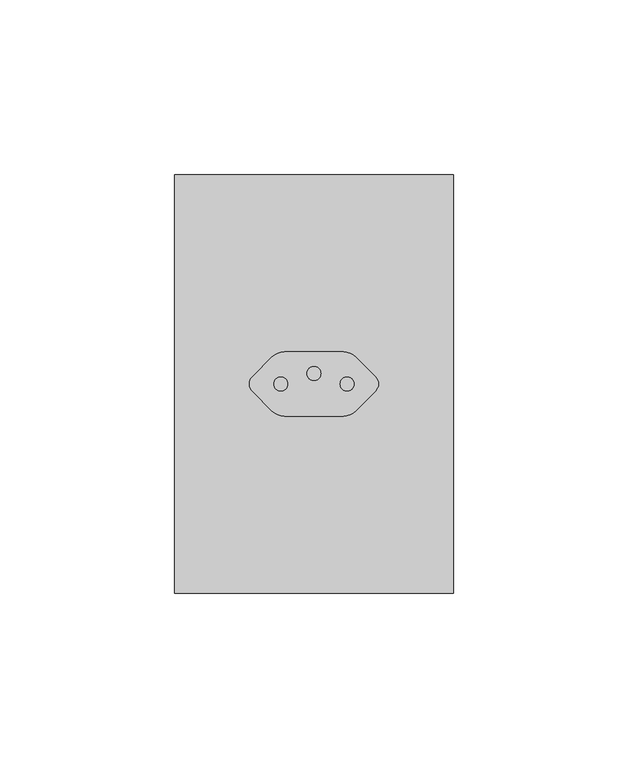
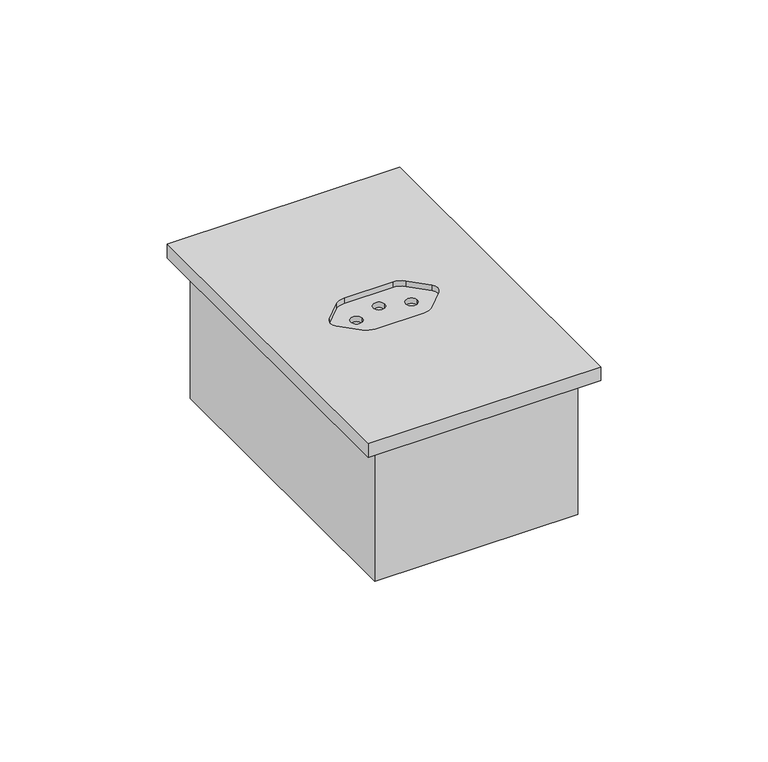
"""IFC4 building model written with IfcOpenShell, lengths in millimetres: proxy geometry, CAIXA VERTICE V7 : Tomada 10A 1s."""

from ifc_helpers import new_model, si_unit, frame, origin, place, context, project, spatial, polyline, circle_curve, faceted_brep, source, transform, mapped, element, save
from ifc_brep_helpers import plane_surface, revolved_surface, advanced_brep


def electrical_fixtures_69341c80(model_context):
    return source(origin(), model_context, "Body", "SolidModel", [
        faceted_brep([(35.0, 355.0, 0.0), (-35.0, 355.0, 0.0), (-35.0, 245.0, 0.0), (35.0, 245.0, 0.0), (33.0, 353.0, 0.0), (33.0, 247.0, 0.0), (-33.0, 247.0, 0.0), (-33.0, 353.0, 0.0), (33.0, 247.0, -48.0), (33.0, 353.0, -48.0), (-33.0, 353.0, -48.0), (-33.0, 247.0, -48.0), (35.0, 355.0, -50.0), (35.0, 245.0, -50.0), (-35.0, 245.0, -50.0), (-35.0, 355.0, -50.0)], [[[0, 1, 2, 3], [4, 5, 6, 7]], [[8, 9, 10, 11]], [[12, 13, 14, 15]], [[12, 15, 1, 0]], [[1, 15, 14, 2]], [[2, 14, 13, 3]], [[3, 13, 12, 0]], [[5, 4, 9, 8]], [[6, 5, 8, 11]], [[7, 6, 11, 10]], [[4, 7, 10, 9]]]),
        advanced_brep(
        [(40.0, 360.0, 5.0), (-40.0, 360.0, 5.0), (-40.0, 240.0, 5.0), (40.0, 240.0, 5.0), (8.4215729, 290.75, 5.0), (-8.4215729, 290.75, 5.0), (-11.9571068, 292.2144661, 5.0), (-17.6213203, 297.8786797, 5.0), (-17.6213203, 302.1213203, 5.0), (-11.9571068, 307.7855339, 5.0), (-8.4215729, 309.25, 5.0), (8.4215729, 309.25, 5.0), (11.9571068, 307.7855339, 5.0), (17.6213203, 302.1213203, 5.0), (17.6213203, 297.8786797, 5.0), (11.9571068, 292.2144661, 5.0), (-40.0, 360.0, 0.0), (40.0, 360.0, 0.0), (40.0, 240.0, 0.0), (-40.0, 240.0, 0.0), (8.4215729, 290.75, 3.0), (11.9571068, 292.2144661, 3.0), (17.6213203, 297.8786797, 3.0), (17.6213203, 302.1213203, 3.0), (11.9571068, 307.7855339, 3.0), (8.4215729, 309.25, 3.0), (-8.4215729, 309.25, 3.0), (-11.9571068, 307.7855339, 3.0), (-17.6213203, 302.1213203, 3.0), (-17.6213203, 297.8786797, 3.0), (-11.9571068, 292.2144661, 3.0), (-8.4215729, 290.75, 3.0), (-7.5, 300.0, 3.0), (-11.5, 300.0, 3.0), (11.5, 300.0, 3.0), (7.5, 300.0, 3.0), (2.0, 303.0, 3.0), (-2.0, 303.0, 3.0), (-11.5, 300.0, 1.0), (-7.5, 300.0, 1.0), (7.5, 300.0, 1.0), (11.5, 300.0, 1.0), (-2.0, 303.0, 1.0), (2.0, 303.0, 1.0)],
        [
            (0, 1),
            (1, 2),
            (2, 3),
            (3, 0),
            (4, 5),
            (5, 6, circle_curve(frame((-8.4215729, 295.75, 5.0), z_axis=(0.0, 0.0, -1.0), x_axis=(-1.0, 0.0, 0.0)), 5.0)),
            (6, 7),
            (7, 8, circle_curve(frame((-15.5, 300.0, 5.0), z_axis=(0.0, 0.0, -1.0), x_axis=(-1.0, 0.0, 0.0)), 3.0)),
            (8, 9),
            (9, 10, circle_curve(frame((-8.4215729, 304.25, 5.0), z_axis=(0.0, 0.0, -1.0), x_axis=(-1.0, 0.0, 0.0)), 5.0)),
            (10, 11),
            (11, 12, circle_curve(frame((8.4215729, 304.25, 5.0), z_axis=(0.0, 0.0, -1.0), x_axis=(-1.0, 0.0, 0.0)), 5.0)),
            (12, 13),
            (13, 14, circle_curve(frame((15.5, 300.0, 5.0), z_axis=(0.0, 0.0, -1.0), x_axis=(-1.0, 0.0, 0.0)), 3.0)),
            (14, 15),
            (15, 4, circle_curve(frame((8.4215729, 295.75, 5.0), z_axis=(0.0, 0.0, -1.0), x_axis=(-1.0, 0.0, 0.0)), 5.0)),
            (16, 17),
            (17, 18),
            (18, 19),
            (19, 16),
            (0, 17),
            (16, 1),
            (19, 2),
            (18, 3),
            (20, 21, circle_curve(frame((8.4215729, 295.75, 3.0), z_axis=(0.0, 0.0, 1.0), x_axis=(-1.0, 0.0, 0.0)), 5.0)),
            (21, 22),
            (22, 23, circle_curve(frame((15.5, 300.0, 3.0), z_axis=(0.0, 0.0, 1.0), x_axis=(-1.0, 0.0, 0.0)), 3.0)),
            (23, 24),
            (24, 25, circle_curve(frame((8.4215729, 304.25, 3.0), z_axis=(0.0, 0.0, 1.0), x_axis=(-1.0, 0.0, 0.0)), 5.0)),
            (25, 26),
            (26, 27, circle_curve(frame((-8.4215729, 304.25, 3.0), z_axis=(0.0, 0.0, 1.0), x_axis=(-1.0, 0.0, 0.0)), 5.0)),
            (27, 28),
            (28, 29, circle_curve(frame((-15.5, 300.0, 3.0), z_axis=(0.0, 0.0, 1.0), x_axis=(-1.0, 0.0, 0.0)), 3.0)),
            (29, 30),
            (30, 31, circle_curve(frame((-8.4215729, 295.75, 3.0), z_axis=(0.0, 0.0, 1.0), x_axis=(-1.0, 0.0, 0.0)), 5.0)),
            (31, 20),
            (32, 33, circle_curve(frame((-9.5, 300.0, 3.0), z_axis=(0.0, 0.0, -1.0), x_axis=(1.0, 2.301812013077709e-12, 0.0)), 2.0)),
            (33, 32, circle_curve(frame((-9.5, 300.0, 3.0), z_axis=(0.0, 0.0, -1.0), x_axis=(1.0, 2.301812013077709e-12, 0.0)), 2.0)),
            (34, 35, circle_curve(frame((9.5, 300.0, 3.0), z_axis=(0.0, 0.0, -1.0), x_axis=(1.0, 2.301812013077709e-12, 0.0)), 2.0)),
            (35, 34, circle_curve(frame((9.5, 300.0, 3.0), z_axis=(0.0, 0.0, -1.0), x_axis=(1.0, 2.301812013077709e-12, 0.0)), 2.0)),
            (36, 37, circle_curve(frame((0.0, 303.0, 3.0), z_axis=(0.0, 0.0, -1.0), x_axis=(1.0, 2.301812013077709e-12, 0.0)), 2.0)),
            (37, 36, circle_curve(frame((0.0, 303.0, 3.0), z_axis=(0.0, 0.0, -1.0), x_axis=(1.0, 2.301812013077709e-12, 0.0)), 2.0)),
            (31, 5),
            (4, 20),
            (30, 6),
            (29, 7),
            (28, 8),
            (27, 9),
            (26, 10),
            (25, 11),
            (24, 12),
            (23, 13),
            (22, 14),
            (21, 15),
            (38, 39, circle_curve(frame((-9.5, 300.0, 1.0), z_axis=(0.0, 0.0, 1.0), x_axis=(1.0, 2.301812013077709e-12, 0.0)), 2.0)),
            (39, 38, circle_curve(frame((-9.5, 300.0, 1.0), z_axis=(0.0, 0.0, 1.0), x_axis=(1.0, 2.301812013077709e-12, 0.0)), 2.0)),
            (40, 41, circle_curve(frame((9.5, 300.0, 1.0), z_axis=(0.0, 0.0, 1.0), x_axis=(1.0, 2.301812013077709e-12, 0.0)), 2.0)),
            (41, 40, circle_curve(frame((9.5, 300.0, 1.0), z_axis=(0.0, 0.0, 1.0), x_axis=(1.0, 2.301812013077709e-12, 0.0)), 2.0)),
            (42, 43, circle_curve(frame((0.0, 303.0, 1.0), z_axis=(0.0, 0.0, 1.0), x_axis=(1.0, 2.301812013077709e-12, 0.0)), 2.0)),
            (43, 42, circle_curve(frame((0.0, 303.0, 1.0), z_axis=(0.0, 0.0, 1.0), x_axis=(1.0, 2.301812013077709e-12, 0.0)), 2.0)),
            (32, 39),
            (38, 33),
            (34, 41),
            (40, 35),
            (36, 43),
            (42, 37),
        ],
        [
            plane_surface(frame((-60.0, 360.0, 5.0), z_axis=(0.0, 0.0, 1.0), x_axis=(-1.0, 0.0, 0.0))),
            plane_surface(frame((-60.0, 360.0, 0.0), z_axis=(0.0, 0.0, -1.0), x_axis=(1.0, 0.0, 0.0))),
            plane_surface(frame((40.0, 360.0, 5.0), z_axis=(0.0, 1.0, 0.0), x_axis=(0.0, 0.0, -1.0))),
            plane_surface(frame((-40.0, 360.0, 5.0), z_axis=(-1.0, 0.0, 0.0), x_axis=(0.0, 0.0, -1.0))),
            plane_surface(frame((-40.0, 240.0, 5.0), z_axis=(0.0, -1.0, 0.0), x_axis=(0.0, 0.0, -1.0))),
            plane_surface(frame((40.0, 240.0, 5.0), z_axis=(1.0, 0.0, 0.0), x_axis=(0.0, 0.0, -1.0))),
            plane_surface(frame((3.4215729, 295.75, 3.0), z_axis=(0.0, 0.0, 1.0), x_axis=(0.0, 1.0, 0.0))),
            plane_surface(frame((-8.4215729, 290.75, 5.0), z_axis=(0.0, 1.0, 0.0), x_axis=(0.0, 0.0, -1.0))),
            revolved_surface(polyline([(-13.4215729, 295.75, 5.0), (-13.4215729, 295.75, 3.0)]), (-8.4215729, 295.75, 3.0), (0.0, 0.0, 1.0)),
            plane_surface(frame((-17.6213203, 297.8786797, 5.0), z_axis=(0.7071067811865045, 0.7071067811865905, 0.0), x_axis=(0.0, 0.0, -1.0))),
            revolved_surface(polyline([(-18.5, 300.0, 5.0), (-18.5, 300.0, 3.0)]), (-15.5, 300.0, 3.0), (0.0, 0.0, 1.0)),
            plane_surface(frame((-11.9571068, 307.7855339, 5.0), z_axis=(0.7071067811865515, -0.7071067811865437, 0.0), x_axis=(0.0, 0.0, -1.0))),
            revolved_surface(polyline([(-13.4215729, 304.25, 5.0), (-13.4215729, 304.25, 3.0)]), (-8.4215729, 304.25, 3.0), (0.0, 0.0, 1.0)),
            plane_surface(frame((8.4215729, 309.25, 5.0), z_axis=(0.0, -1.0, 0.0), x_axis=(0.0, 0.0, -1.0))),
            revolved_surface(polyline([(3.4215728999999993, 304.25, 5.0), (3.4215728999999993, 304.25, 3.0)]), (8.4215729, 304.25, 3.0), (0.0, 0.0, 1.0)),
            plane_surface(frame((17.6213203, 302.1213203, 5.0), z_axis=(-0.7071067811865307, -0.7071067811865643, 0.0), x_axis=(0.0, 0.0, -1.0))),
            revolved_surface(polyline([(12.5, 300.0, 5.0), (12.5, 300.0, 3.0)]), (15.5, 300.0, 3.0), (0.0, 0.0, 1.0)),
            plane_surface(frame((11.9571068, 292.2144661, 5.0), z_axis=(-0.7071067811865893, 0.7071067811865058, 0.0), x_axis=(0.0, 0.0, -1.0))),
            revolved_surface(polyline([(3.4215728999999993, 295.75, 5.0), (3.4215728999999993, 295.75, 3.0)]), (8.4215729, 295.75, 3.0), (0.0, 0.0, 1.0)),
            plane_surface(frame((-7.5, 300.0, 1.0), z_axis=(0.0, 0.0, 1.0), x_axis=(2.301812013077709e-12, -1.0, 0.0))),
            revolved_surface(polyline([(-7.5, 300.0000000000046, 3.0), (-7.5, 300.0000000000046, 1.0)]), (-9.5, 300.0, 1.0), (0.0, 0.0, 1.0)),
            revolved_surface(polyline([(11.5, 300.0000000000046, 3.0), (11.5, 300.0000000000046, 1.0)]), (9.5, 300.0, 5.0), (0.0, 0.0, 1.0)),
            revolved_surface(polyline([(2.0, 303.0000000000046, 3.0), (2.0, 303.0000000000046, 1.0)]), (0.0, 303.0, 5.0), (0.0, 0.0, 1.0)),
        ],
        [
            (0, [[1, 2, 3, 4], [5, 6, 7, 8, 9, 10, 11, 12, 13, 14, 15, 16]]),
            (1, [[17, 18, 19, 20]]),
            (2, [[-1, 21, -17, 22]]),
            (3, [[-2, -22, -20, 23]]),
            (4, [[-3, -23, -19, 24]]),
            (5, [[-4, -24, -18, -21]]),
            (6, [[25, 26, 27, 28, 29, 30, 31, 32, 33, 34, 35, 36], [37, 38], [39, 40], [41, 42]]),
            (7, [[-36, 43, -5, 44]]),
            (8, [[-35, 45, -6, -43]]),
            (9, [[-34, 46, -7, -45]]),
            (10, [[-33, 47, -8, -46]]),
            (11, [[-32, 48, -9, -47]]),
            (12, [[-31, 49, -10, -48]]),
            (13, [[-30, 50, -11, -49]]),
            (14, [[-29, 51, -12, -50]]),
            (15, [[-28, 52, -13, -51]]),
            (16, [[-27, 53, -14, -52]]),
            (17, [[-26, 54, -15, -53]]),
            (18, [[-25, -44, -16, -54]]),
            (19, [[55, 56]]),
            (19, [[57, 58]]),
            (19, [[59, 60]]),
            (20, [[-37, 61, -55, 62]]),
            (20, [[-38, -62, -56, -61]]),
            (21, [[-39, 63, -57, 64]]),
            (21, [[-40, -64, -58, -63]]),
            (22, [[-41, 65, -59, 66]]),
            (22, [[-42, -66, -60, -65]]),
        ],
    ),
    ])


if __name__ == "__main__":
    model = new_model("IFC4")
    model_context = context("Model", 3, world=origin())
    ifc_project = project(units=[si_unit("LENGTHUNIT", "METRE", prefix="MILLI")], contexts=[model_context])
    site = spatial("IfcSite", under=ifc_project)
    building = spatial("IfcBuilding", under=site)
    placement = place(None, origin())
    electrical_fixtures_shape = electrical_fixtures_69341c80(model_context)
    element("IfcBuildingElementProxy", 1, Name="CAIXA VERTICE V7 : Tomada 10A 1s", ObjectType="CAIXA VERTICE V7 : Tomada 10A 1s", at=placement, inside=building, context=model_context, shape_type="MappedRepresentation", body=[
        mapped(electrical_fixtures_shape, transform((0.0, 0.0, 0.0), x_axis=(1.0, 0.0, 0.0), y_axis=(0.0, 1.0, 0.0), z_axis=(0.0, 0.0, 1.0))),
    ])
    save(model, "model.ifc")

# Revit data of these elements
# Type "CAIXA VERTICE V7 : Tomada 10A 1s"
#   URL = "www.facebook.com/verticetreinamentos"
#   SEÇÃO [instance default] = ""
#   Rotação [instance default] = 0.00°
#   LARGURA DA TAMPA = 0.08 m
#   BORDA = 0.01 m
#   ALTURA DE INSTALAÇÃO [instance default] = 1.10 m
#   Distância Anotação [instance default] = 0.0015 m
#   ALTURA DA TAMPA = 0.12 m
#   Vertical [instance default] = yes
#   VER SEÇÃO [instance default] = no
#   SHADE ESQ [instance default] = no
#   SHADE DIR [instance default] = yes
#   HORIZONTAL [instance default] = no
#   ANDAR COM A LEGENDA [instance default] = 0
#   Material Tampa [instance default] = Plástico, branco opaco
#   Caixa = element 1798514
#   Anotação = element 1798528
#   Default Elevation = 0
# Element 1 (IfcBuildingElementProxy, "CAIXA VERTICE V7 : Tomada 10A 1s")
#   ALTURA DE INSTALAÇÃO = 0.30 m
#   SHADE DIR = no
#   Materials on its faces: "Plástico, branco opaco"
# Materials
#   "Plástico, branco opaco": class "Plástico", colour RGB 120 120 120, transparency 0, Description = "Plastic, generic, opaque white", Cost = 0
